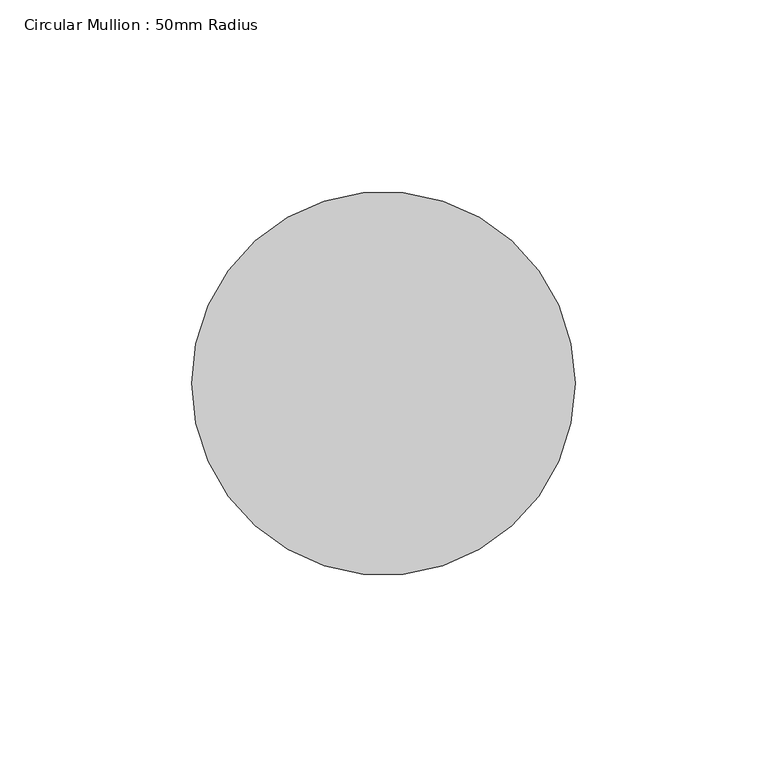
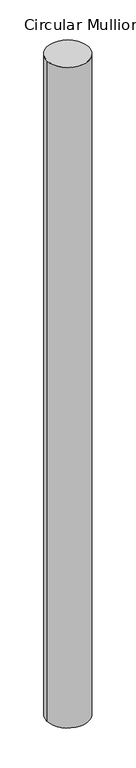
"""IFC4 building model written with IfcOpenShell, lengths in millimetres: member geometry, Circular Mullion : 50mm Radius."""

from ifc_helpers import new_model, si_unit, point, frame, origin, origin_2d, place, context, project, spatial, circle_curve, trimmed, segment, composite_curve, outline, extrude, source, transform, mapped, element, save


def circular_mullion_50mm_radius_7f7191f1(model_context):
    return source(origin(), model_context, "Body", "SweptSolid", [
        extrude(outline(composite_curve([segment(trimmed(circle_curve(origin_2d(), 50.0), [point((50.0, 0.0))], [point((-50.0, 0.0))], False, "CARTESIAN"), True, "CONTINUOUS"), segment(trimmed(circle_curve(origin_2d(), 50.0), [point((-50.0, 0.0))], [point((50.0, 0.0))], False, "CARTESIAN"), True, "CONTINUOUS")], self_intersect=False)), frame((0.0, 0.0, -1674.1937508), z_axis=(0.0, 0.0, 1.0), x_axis=(1.0, 0.0, 0.0)), (0.0, 0.0, 1.0), 1674.1937508),
    ])


if __name__ == "__main__":
    model = new_model("IFC4")
    model_context = context("Model", 3, world=origin())
    ifc_project = project(units=[si_unit("LENGTHUNIT", "METRE", prefix="MILLI")], contexts=[model_context])
    site = spatial("IfcSite", under=ifc_project)
    building = spatial("IfcBuilding", under=site)
    placement = place(None, origin())
    circular_mullion_50mm_radius_shape = circular_mullion_50mm_radius_7f7191f1(model_context)
    element("IfcMember", 1, ObjectType="Circular Mullion : 50mm Radius", at=placement, inside=building, context=model_context, shape_type="MappedRepresentation", body=[
        mapped(circular_mullion_50mm_radius_shape, transform((0.0, 0.0, 0.0), x_axis=(1.0, 0.0, 0.0), y_axis=(0.0, 1.0, 0.0), z_axis=(0.0, 0.0, 1.0))),
    ])
    save(model, "model.ifc")

# Revit data of these elements
# Type "Circular Mullion : 50mm Radius"
#   built-in parameter 1007350 = 0.164042 (stored number, unit not read)
# Element 1 (IfcMember, "Circular Mullion : 50mm Radius")
#   Materials on its faces: "Aluminium"
# Materials
#   "Aluminium": class "Metal", colour RGB 247 247 247, transparency 0, Description = "Aluminium 6061", Cost = 0
